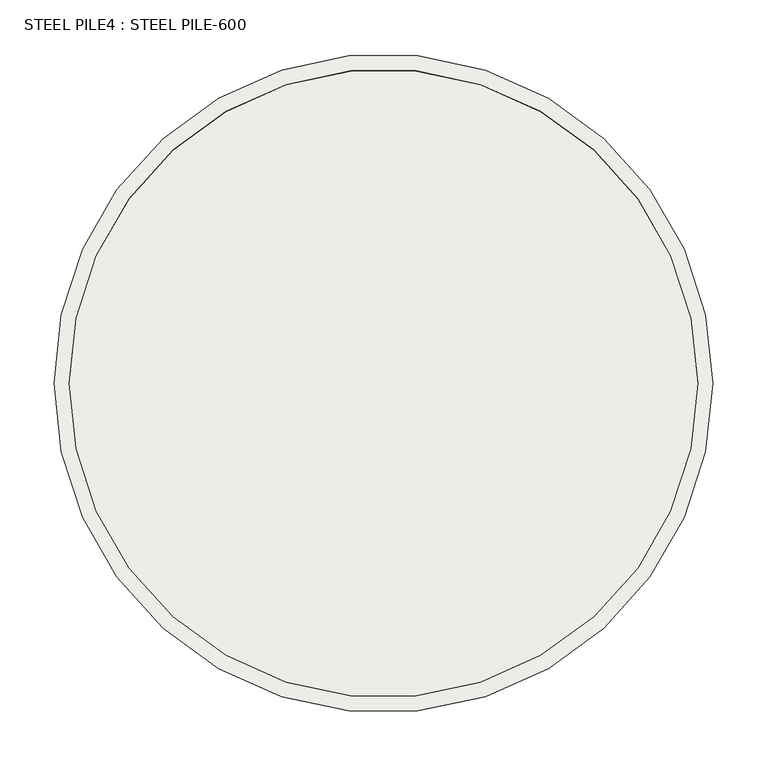
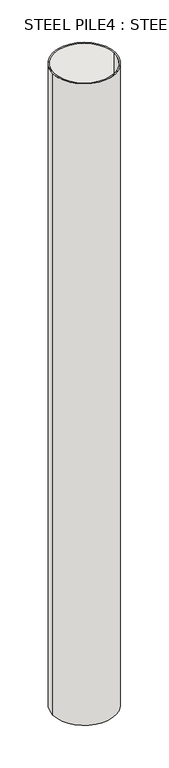
"""IFC4 building model written with IfcOpenShell, lengths in millimetres: slab geometry, STEEL PILE4 : STEEL PILE-600."""

from ifc_helpers import new_model, si_unit, point, frame, frame_2d, origin, place, context, project, spatial, circle_curve, trimmed, segment, composite_curve, outline, extrude, source, transform, mapped, element, save


def steel_pile4_steel_pile_600_1e1ce682(model_context):
    return source(origin(), model_context, "Body", "SweptSolid", [
        extrude(outline(composite_curve([segment(trimmed(circle_curve(frame_2d((7920.0, 66679.5208589)), 290.5), [point((7629.5, 66679.5208589))], [point((8210.5, 66679.5208589))], False, "CARTESIAN"), True, "CONTINUOUS"), segment(trimmed(circle_curve(frame_2d((7920.0, 66679.5208589)), 290.5), [point((8210.5, 66679.5208589))], [point((7629.5, 66679.5208589))], False, "CARTESIAN"), True, "CONTINUOUS")], self_intersect=False)), frame((0.0, 0.0, -2530.0), z_axis=(0.0, 0.0, 1.0), x_axis=(1.0, 0.0, 0.0)), (0.0, 0.0, 1.0), 30.0),
        extrude(outline(composite_curve([segment(trimmed(circle_curve(frame_2d((7920.0, 66679.5208589)), 304.5), [point((7615.5, 66679.5208589))], [point((8224.5, 66679.5208589))], False, "CARTESIAN"), True, "CONTINUOUS"), segment(trimmed(circle_curve(frame_2d((7920.0, 66679.5208589)), 304.5), [point((8224.5, 66679.5208589))], [point((7615.5, 66679.5208589))], False, "CARTESIAN"), True, "CONTINUOUS")], self_intersect=False), holes=[composite_curve([segment(trimmed(circle_curve(frame_2d((7920.0, 66679.5208589)), 290.5), [point((7629.5, 66679.5208589))], [point((8210.5, 66679.5208589))], True, "CARTESIAN"), True, "CONTINUOUS"), segment(trimmed(circle_curve(frame_2d((7920.0, 66679.5208589)), 290.5), [point((8210.5, 66679.5208589))], [point((7629.5, 66679.5208589))], True, "CARTESIAN"), True, "CONTINUOUS")], self_intersect=False)]), frame((0.0, 0.0, -7500.0), z_axis=(0.0, 0.0, 1.0), x_axis=(1.0, 0.0, 0.0)), (0.0, 0.0, 1.0), 6600.0),
    ])


if __name__ == "__main__":
    model = new_model("IFC4")
    model_context = context("Model", 3, world=origin())
    ifc_project = project(units=[si_unit("LENGTHUNIT", "METRE", prefix="MILLI")], contexts=[model_context])
    site = spatial("IfcSite", under=ifc_project)
    building = spatial("IfcBuilding", under=site)
    placement = place(None, origin())
    steel_pile4_steel_pile_600_shape = steel_pile4_steel_pile_600_1e1ce682(model_context)
    element("IfcSlab", 1, ObjectType="STEEL PILE4 : STEEL PILE-600", at=placement, inside=building, context=model_context, shape_type="MappedRepresentation", body=[
        mapped(steel_pile4_steel_pile_600_shape, transform((0.0, 0.0, 0.0), x_axis=(1.0, 0.0, 0.0), y_axis=(0.0, 1.0, 0.0), z_axis=(0.0, 0.0, 1.0))),
    ])
    save(model, "model.ifc")

# Revit data of these elements
# Element 1 (IfcSlab, "STEEL PILE4 : STEEL PILE-600")
#   Materials on its faces: "Metal - Steel"
# Materials
#   "Metal - Steel": class "Metal", colour RGB 247 247 247, transparency 0, Cost = 0
